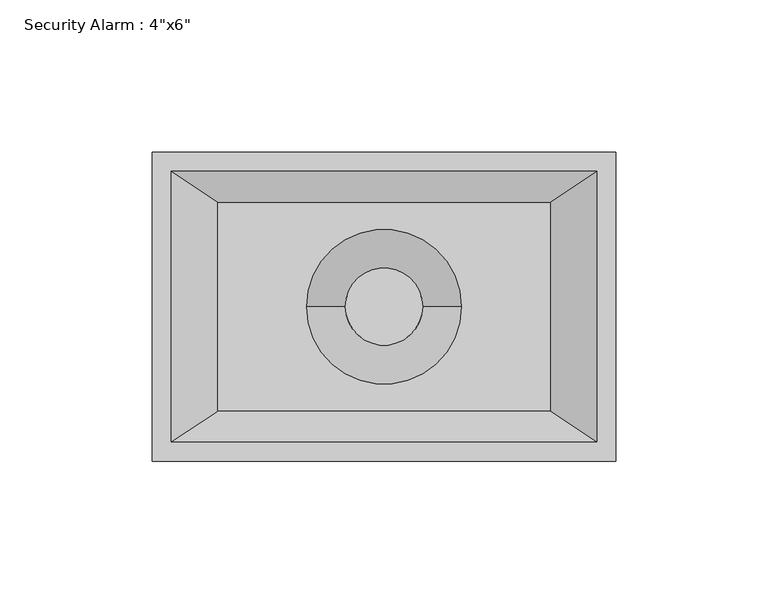
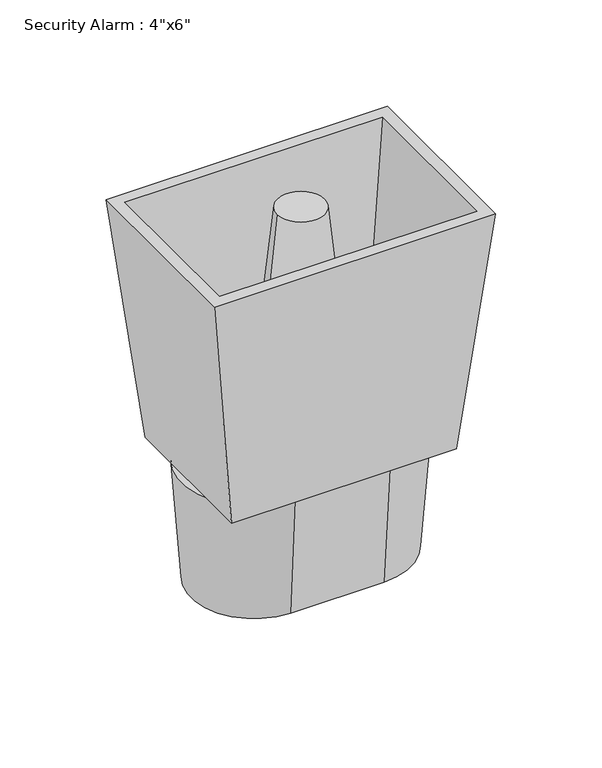
"""IFC4 building model written with IfcOpenShell, lengths in millimetres: proxy geometry."""

from ifc_helpers import new_model, si_unit, frame, origin, place, context, project, spatial, polyline, circle_curve, faceted_brep, source, transform, mapped, element, save
from ifc_brep_helpers import plane_surface, revolved_surface, spline_surface, advanced_brep


def proxy_189e13d4(model_context):
    return source(origin(), model_context, "Body", "SolidModel", [
        faceted_brep([(76.2, 50.8, 203.2), (-76.2, 50.8, 203.2), (-76.2, -50.8, 203.2), (76.2, -50.8, 203.2), (-69.85, 44.45, 203.2), (69.85, 44.45, 203.2), (69.85, -44.45, 203.2), (-69.85, -44.45, 203.2), (60.96, 40.64, 67.7333333), (60.96, -40.64, 67.7333333), (-60.96, -40.64, 67.7333333), (-60.96, 40.64, 67.7333333), (54.61, 34.29, 74.0833333), (-54.61, 34.29, 74.0833333), (-54.61, -34.29, 74.0833333), (54.61, -34.29, 74.0833333)], [[[0, 1, 2, 3], [4, 5, 6, 7]], [[8, 9, 10, 11]], [[1, 0, 8, 11]], [[2, 1, 11, 10]], [[3, 2, 10, 9]], [[0, 3, 9, 8]], [[12, 13, 14, 15]], [[13, 12, 5, 4]], [[14, 13, 4, 7]], [[15, 14, 7, 6]], [[12, 15, 6, 5]]]),
        advanced_brep(
        [(-12.7, 0.0, 203.2), (12.7, 0.0, 203.2), (-25.4, 0.0, 80.4333333), (25.4, 0.0, 80.4333333)],
        [
            (0, 1, circle_curve(frame((0.0, 0.0, 203.2), z_axis=(0.0, 0.0, 1.0), x_axis=(-1.0, 0.0, 0.0)), 12.7)),
            (1, 0, circle_curve(frame((0.0, 0.0, 203.2), z_axis=(0.0, 0.0, 1.0), x_axis=(1.0, 0.0, 0.0)), 12.7)),
            (2, 3, circle_curve(frame((0.0, 0.0, 80.4333333), z_axis=(0.0, 0.0, -1.0), x_axis=(1.0, 0.0, 0.0)), 25.4)),
            (3, 2, circle_curve(frame((0.0, 0.0, 80.4333333), z_axis=(0.0, 0.0, -1.0), x_axis=(-1.0, 0.0, 0.0)), 25.4)),
            (3, 1),
            (0, 2),
        ],
        [
            plane_surface(frame((0.0, 0.0, 203.2), z_axis=(0.0, 0.0, 1.0), x_axis=(0.0, -1.0, 0.0))),
            plane_surface(frame((0.0, 0.0, 80.4333333), z_axis=(0.0, 0.0, -1.0), x_axis=(0.0, -1.0, 0.0))),
            revolved_surface(polyline([(-12.700000000000003, 0.0, 203.2), (-25.4, 0.0, 80.43333330000002)]), (0.0, 0.0, 325.9666667), (0.0, 0.0, -1.0)),
            revolved_surface(polyline([(12.700000000000003, 0.0, 203.2), (25.4, 0.0, 80.43333330000002)]), (0.0, 0.0, 325.9666667), (0.0, 0.0, -1.0)),
        ],
        [
            (0, [[1, 2]]),
            (1, [[3, 4]]),
            (2, [[-4, 5, -1, 6]]),
            (3, [[-3, -6, -2, -5]]),
        ],
    ),
        advanced_brep(
        [(25.7175, 39.0525, 67.7333333), (-25.7175, 39.0525, 67.7333333), (-25.7175, -39.0525, 67.7333333), (25.7175, -39.0525, 67.7333333), (25.4, 34.29, 0.0), (25.4, -34.29, 0.0), (-25.4, -34.29, 0.0), (-25.4, 34.29, 0.0)],
        [
            (0, 1),
            (1, 2, circle_curve(frame((-25.7175, 0.0, 67.7333333), z_axis=(0.0, 0.0, 1.0), x_axis=(1.0, 0.0, 0.0)), 39.0525)),
            (2, 3),
            (3, 0, circle_curve(frame((25.7175, 0.0, 67.7333333), z_axis=(0.0, 0.0, 1.0), x_axis=(1.0, 0.0, 0.0)), 39.0525)),
            (4, 5, circle_curve(frame((25.4, 0.0, 0.0), z_axis=(0.0, 0.0, -1.0), x_axis=(1.0, 0.0, 0.0)), 34.29)),
            (5, 6),
            (6, 7, circle_curve(frame((-25.4, 0.0, 0.0), z_axis=(0.0, 0.0, -1.0), x_axis=(1.0, 0.0, 0.0)), 34.29)),
            (7, 4),
            (7, 1),
            (0, 4),
            (6, 2),
            (5, 3),
        ],
        [
            plane_surface(frame((0.0, 0.0, 67.7333333), z_axis=(0.0, 0.0, 1.0), x_axis=(1.0, 0.0, 0.0))),
            plane_surface(frame((0.0, 0.0, 0.0), z_axis=(0.0, 0.0, -1.0), x_axis=(1.0, 0.0, 0.0))),
            plane_surface(frame((0.0, 34.29, 0.0), z_axis=(0.0, 0.9975372041844565, -0.07013933466934312), x_axis=(-1.0, 0.0, 0.0))),
            spline_surface(2, 1, [[(-25.4, 34.29, 0.0), (-25.7175, 39.0525, 67.7333333)], [(-59.69, 34.29, 0.0), (-64.77000000000001, 39.0525, 67.7333333)], [(-59.69, 0.0, 0.0), (-64.77000000000001, 0.0, 67.7333333)], [(-59.69, -34.29, 0.0), (-64.77000000000001, -39.0525, 67.7333333)], [(-25.4, -34.29, 0.0), (-25.7175, -39.0525, 67.7333333)]], [3, 2, 3], [2, 2], [0.0, 1.0, 2.0], [0.0, 1.0], weights=[[1.0, 1.0], [0.7071067811865476, 0.7071067811865476], [1.0, 1.0], [0.7071067811865476, 0.7071067811865476], [1.0, 1.0]]),
            plane_surface(frame((0.0, -34.29, 0.0), z_axis=(0.0, -0.9975372041844384, -0.07013933466960001), x_axis=(1.0, 0.0, 0.0))),
            spline_surface(2, 1, [[(25.4, -34.29, 0.0), (25.7175, -39.0525, 67.7333333)], [(59.69, -34.29, 0.0), (64.77000000000001, -39.0525, 67.7333333)], [(59.69, 0.0, 0.0), (64.77000000000001, 0.0, 67.7333333)], [(59.69, 34.29, 0.0), (64.77000000000001, 39.0525, 67.7333333)], [(25.4, 34.29, 0.0), (25.7175, 39.0525, 67.7333333)]], [3, 2, 3], [2, 2], [0.0, 1.0, 2.0], [0.0, 1.0], weights=[[1.0, 1.0], [0.7071067811865476, 0.7071067811865476], [1.0, 1.0], [0.7071067811865476, 0.7071067811865476], [1.0, 1.0]]),
        ],
        [
            (0, [[1, 2, 3, 4]]),
            (1, [[5, 6, 7, 8]]),
            (2, [[-8, 9, -1, 10]]),
            (3, [[-7, 11, -2, -9]]),
            (4, [[-6, 12, -3, -11]]),
            (5, [[-5, -10, -4, -12]]),
        ],
    ),
    ])


if __name__ == "__main__":
    model = new_model("IFC4")
    model_context = context("Model", 3, world=origin())
    ifc_project = project(units=[si_unit("LENGTHUNIT", "METRE", prefix="MILLI")], contexts=[model_context])
    site = spatial("IfcSite", under=ifc_project)
    building = spatial("IfcBuilding", under=site)
    placement = place(None, origin())
    proxy_shape = proxy_189e13d4(model_context)
    element("IfcBuildingElementProxy", 1, Name="Security Alarm : 4\"x6\"", ObjectType="Security Alarm : 4\"x6\"", at=placement, inside=building, context=model_context, shape_type="MappedRepresentation", body=[
        mapped(proxy_shape, transform((0.0, 0.0, 0.0), x_axis=(1.0, 0.0, 0.0), y_axis=(0.0, 1.0, 0.0), z_axis=(0.0, 0.0, 1.0))),
    ])
    save(model, "model.ifc")

# Revit data of these elements
# Project information
#   Project Issue Date = "Issue Date"
#   Project Status = "Project Status"
#   Client Name = "Owner"
#   Project Address = "Enter address here"
#   Project Name = "Project Name"
#   Project Number = "Project Number"
# Type "Security Alarm : 4\"x6\""
#   Width 1 = 0' - 3.2"
#   Radius 1 = 0' - 1.6"
#   Length 1 = 0' - 4.8"
#   Height 1 = 0' - 2.66667"
#   Default Elevation = 4' - 0"
#   Siren Width = 0' - 4"
#   Siren Length = 0' - 6"
#   Siren Height = 0' - 8"
#   Siren Material = none
